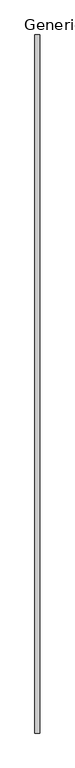
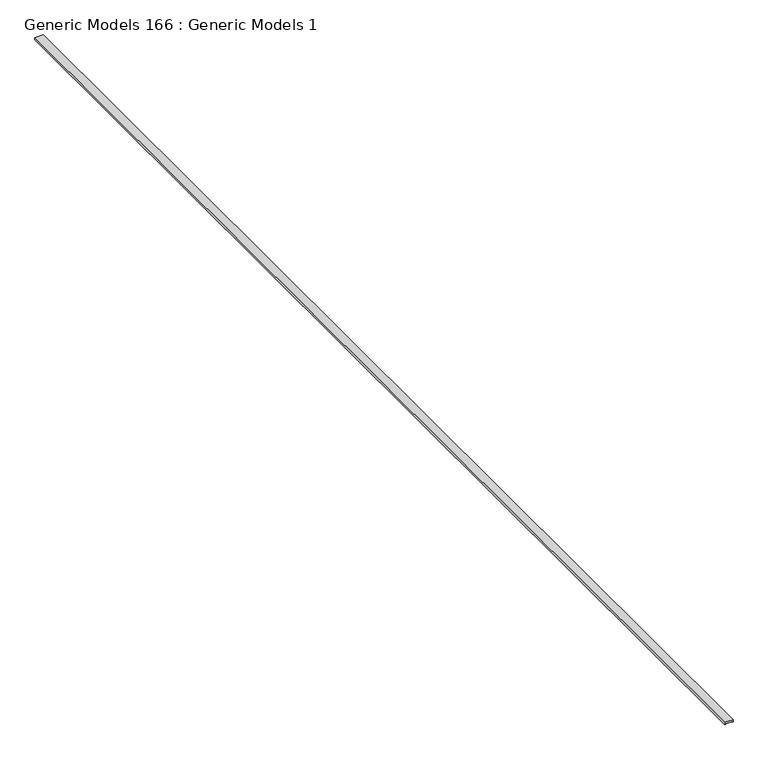
"""IFC4 building model written with IfcOpenShell, lengths in millimetres: proxy geometry, Generic Models 166 : Generic Models 1."""

from ifc_helpers import new_model, si_unit, frame, origin, place, context, project, spatial, polyline, outline, extrude, source, transform, mapped, element, save


def generic_models_166_generic_models_1_49732ac5(model_context):
    return source(origin(), model_context, "Body", "SweptSolid", [
        extrude(outline(polyline([(124147.4242034, -10305.9597239), (124147.4242034, -10372.6347239), (124128.3742034, -10372.6347239), (124128.3742034, -10364.6972239), (124134.7242034, -10364.6972239), (124134.7242034, -10313.8972239), (124128.3742034, -10313.8972239), (124128.3742034, -10305.9597239), (124147.4242034, -10305.9597239)])), frame((0.0, -654.6230338, 0.0), z_axis=(0.0, 1.0, 0.0), x_axis=(0.0, 0.0, 1.0)), (0.0, 0.0, 1.0), 9475.7774227),
    ])


if __name__ == "__main__":
    model = new_model("IFC4")
    model_context = context("Model", 3, world=origin())
    ifc_project = project(units=[si_unit("LENGTHUNIT", "METRE", prefix="MILLI")], contexts=[model_context])
    site = spatial("IfcSite", under=ifc_project)
    building = spatial("IfcBuilding", under=site)
    placement = place(None, origin())
    generic_models_166_generic_models_1_shape = generic_models_166_generic_models_1_49732ac5(model_context)
    element("IfcBuildingElementProxy", 1, Name="Generic Models 166 : Generic Models 1", ObjectType="Generic Models 166 : Generic Models 1", at=placement, inside=building, context=model_context, shape_type="MappedRepresentation", body=[
        mapped(generic_models_166_generic_models_1_shape, transform((0.0, 0.0, 0.0), x_axis=(1.0, 0.0, 0.0), y_axis=(0.0, 1.0, 0.0), z_axis=(0.0, 0.0, 1.0))),
    ])
    save(model, "model.ifc")

# Revit data of these elements
# Element 1 (IfcBuildingElementProxy, "Generic Models 166 : Generic Models 1")
#   Materials on its faces: "_2 5/8\" X 3/4\" WOOD TOP RAIL / HAND RAIL, EASE EDGES W/ .01 RADIUS"
# Materials
#   "_2 5/8\" X 3/4\" WOOD TOP RAIL / HAND RAIL, EASE EDGES W/ .01 RADIUS": class "Generic", colour RGB 177 130 114, transparency 0, Cost = 0
